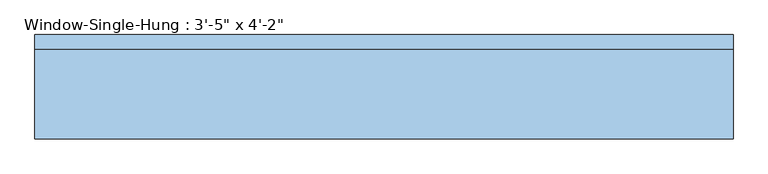
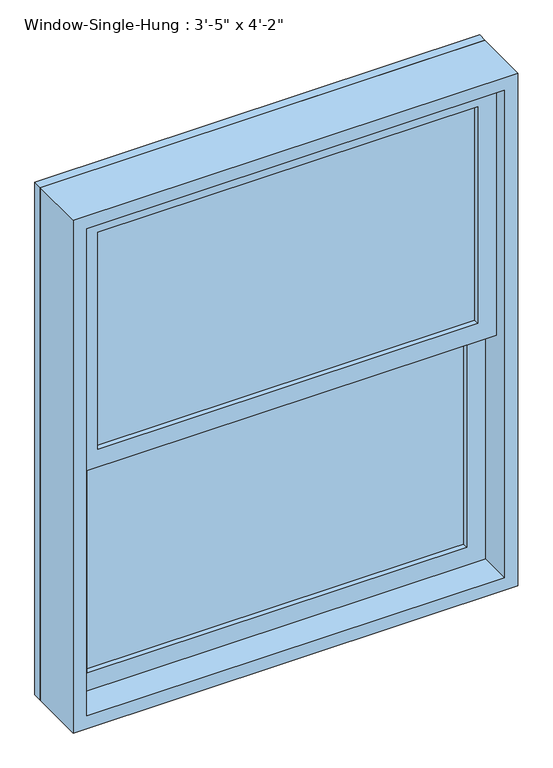
"""IFC4 building model written with IfcOpenShell, lengths in millimetres: window geometry."""

from ifc_helpers import new_model, si_unit, frame, origin, place, context, project, spatial, polyline, outline, extrude, source, transform, mapped, element, save


def window_843688b7(model_context):
    return source(origin(), model_context, "Body", "SweptSolid", [
        extrude(outline(polyline([(444.5, 1.5875), (-444.5, 1.5875), (-444.5, 7.9375), (444.5, 7.9375), (444.5, 1.5875)])), frame((0.0, 0.0, 990.6), z_axis=(0.0, 0.0, 1.0), x_axis=(1.0, 0.0, 0.0)), (0.0, 0.0, 1.0), 536.575),
        extrude(outline(polyline([(-444.5, 14.2875), (-444.5, 20.6375), (444.5, 20.6375), (444.5, 14.2875), (-444.5, 14.2875)])), frame((0.0, 0.0, 990.6), z_axis=(0.0, 0.0, 1.0), x_axis=(1.0, 0.0, 0.0)), (0.0, 0.0, 1.0), 536.575),
        extrude(outline(polyline([(444.5, -42.8625), (-444.5, -42.8625), (-444.5, -36.5125), (444.5, -36.5125), (444.5, -42.8625)])), frame((0.0, 0.0, 1571.625), z_axis=(0.0, 0.0, 1.0), x_axis=(1.0, 0.0, 0.0)), (0.0, 0.0, 1.0), 536.575),
        extrude(outline(polyline([(-444.5, -30.1625), (-444.5, -23.8125), (444.5, -23.8125), (444.5, -30.1625), (-444.5, -30.1625)])), frame((0.0, 0.0, 1571.625), z_axis=(0.0, 0.0, 1.0), x_axis=(1.0, 0.0, 0.0)), (0.0, 0.0, 1.0), 536.575),
        extrude(outline(polyline([(1571.625, 488.95), (1571.625, -488.95), (946.15, -488.95), (946.15, 488.95), (1571.625, 488.95)]), holes=[polyline([(1527.175, -444.5), (1527.175, 444.5), (990.6, 444.5), (990.6, -444.5), (1527.175, -444.5)])]), frame((0.0, -11.1125, 0.0), z_axis=(0.0, 1.0, 0.0), x_axis=(0.0, 0.0, 1.0)), (0.0, 0.0, 1.0), 44.45),
        extrude(outline(polyline([(2152.65, 488.95), (2152.65, -488.95), (1527.175, -488.95), (1527.175, 488.95), (2152.65, 488.95)]), holes=[polyline([(2108.2, -444.5), (2108.2, 444.5), (1571.625, 444.5), (1571.625, -444.5), (2108.2, -444.5)])]), frame((0.0, -55.5625, 0.0), z_axis=(0.0, 1.0, 0.0), x_axis=(0.0, 0.0, 1.0)), (0.0, 0.0, 1.0), 44.45),
        extrude(outline(polyline([(2184.4, 520.7), (2184.4, -520.7), (914.4, -520.7), (914.4, 520.7), (2184.4, 520.7)]), holes=[polyline([(2152.65, -488.95), (2152.65, 488.95), (946.15, 488.95), (946.15, -488.95), (2152.65, -488.95)])]), frame((0.0, -87.3125, 0.0), z_axis=(0.0, 1.0, 0.0), x_axis=(0.0, 0.0, 1.0)), (0.0, 0.0, 1.0), 133.35),
        extrude(outline(polyline([(2184.4, 520.7), (2184.4, -520.7), (914.4, -520.7), (914.4, 520.7), (2184.4, 520.7)]), holes=[polyline([(2165.35, 501.65), (933.45, 501.65), (933.45, -501.65), (2165.35, -501.65), (2165.35, 501.65)])]), frame((0.0, 46.0375, 0.0), z_axis=(0.0, 1.0, 0.0), x_axis=(0.0, 0.0, 1.0)), (0.0, 0.0, 1.0), 22.225),
    ])


if __name__ == "__main__":
    model = new_model("IFC4")
    model_context = context("Model", 3, world=origin())
    ifc_project = project(units=[si_unit("LENGTHUNIT", "METRE", prefix="MILLI")], contexts=[model_context])
    site = spatial("IfcSite", under=ifc_project)
    building = spatial("IfcBuilding", under=site)
    placement = place(None, origin())
    window_shape = window_843688b7(model_context)
    element("IfcWindow", 1, ObjectType="Window-Single-Hung : 3'-5\" x 4'-2\"", at=placement, inside=building, context=model_context, shape_type="MappedRepresentation", body=[
        mapped(window_shape, transform((0.0, 0.0, 0.0), x_axis=(1.0, 0.0, 0.0), y_axis=(0.0, 1.0, 0.0), z_axis=(0.0, 0.0, 1.0))),
    ])
    save(model, "model.ifc")

# Revit data of these elements
# Type "Window-Single-Hung : 3'-5\" x 4'-2\""
#   Type Mark = "24"
#   Fire Rating = "0.5h"
#   Construction Type Id = "DG-DR"
#   Assembly Code = "B2020100"
#   Analytic Construction = "Double glazing - domestic"
#   Wall Thickness [instance default] = 0' - 6"
#   Window Inset [instance default] = 0' - 0"
#   Visual Light Transmittance = 0.81
#   Thermal Resistance (R) = 0.319569 (m²·K)/W
#   Solar Heat Gain Coefficient = 0.76
#   Muntin Width = 2' - 11"
#   Muntin Height = 1' - 9 1/8"
#   Interior Wall Closure [instance default] = 0' - 1 1/2"
#   Rough Width = 3' - 5 1/2"
#   Rough Height = 4' - 2 1/2"
#   Frame Extension [instance default] = 0' - 1 1/4"
#   Exterior Wall Closure [instance default] = 0' - 0 1/2"
#   Extension Jamb [instance default] = 0' - 1 1/2"
#   Heat Transfer Coefficient (U) = 3.12929 W/(m²·K)
#   Height = 4' - 2"
#   Width = 3' - 5"
#   Top Muntin Visibility = yes
#   Indicator Visibility [instance default] = yes
#   Extension Jamb Visibility [instance default] = yes
#   Interior Trim Visibility [instance default] = yes
#   Exterior Trim Visibility [instance default] = yes
#   Bottom Muntin Visibility = yes
#   Muntin Pattern = Muntin Pattern_2x2 : Muntin Pattern_2x2
#   Interior Trim Material = Wood - Stained
#   Interior Trim = Trim-Window-Interior-Flat : Picture Frame
#   Exterior Trim Material = Clad - White
#   Exterior Trim = Trim-Window-Exterior-Flat : with Sill
#   Glass Panel Material = Glass
#   Exterior Frame Material = Clad - White
#   Interior Frame Material = Wood - Stained
#   Wall Closure = (empty or 0)
# Element 1 (IfcWindow, "Window-Single-Hung : 3'-5\" x 4'-2\"")
#   Wall Thickness = 0' - 5 3/8"
#   Extension Jamb = 0' - 0 7/8"
#   Materials on its faces: "Wood - Stained", "Glass", "Clad - White"
# Materials
#   "Wood - Stained": class "Wood", colour RGB 224 178 126, transparency 0, Cost = 0
#   "Clad - White": class "Wood", colour RGB 242 242 238, transparency 0, Cost = 0
#   "Glass": class "Glass", colour RGB 0 128 192, transparency 0.75, Description = "Soda Lime Glass", Cost = 0
